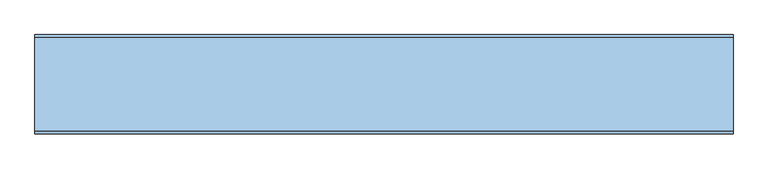
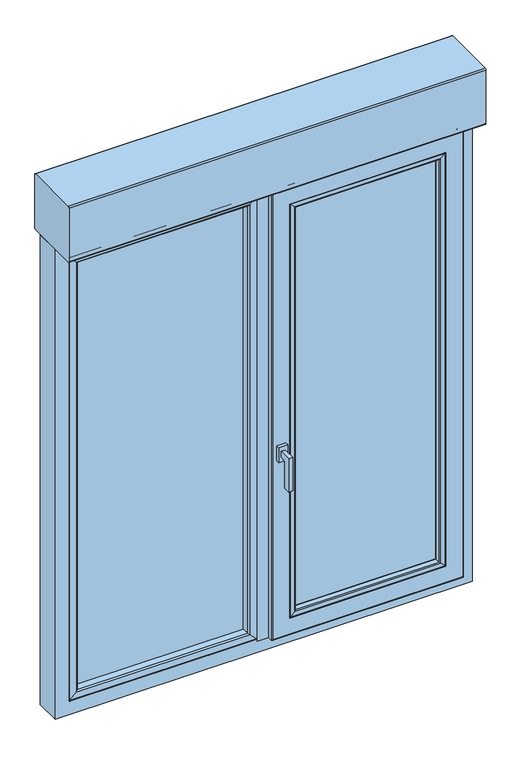
"""IFC4 building model written with IfcOpenShell, lengths in millimetres: window geometry, 2019_ES_Ventana_Replus_re80pvc301_11103_box_1-Hoja_Panel-Fijo-Lateral_con-Compacto : 2019_ES_Ventana_replus_re80pvc_301_dormitorio_1."""

from ifc_helpers import new_model, si_unit, point, frame, frame_2d, origin, place, context, project, spatial, polyline, circle_curve, ellipse_curve, trimmed, segment, composite_curve, outline, extrude, source, transform, mapped, element, save
from ifc_brep_helpers import plane_surface, cylinder_surface, advanced_brep


def window_05755cfc(model_context):
    return source(origin(), model_context, "Body", "SolidModel", [
        extrude(outline(composite_curve([segment(polyline([(55.0, 2360.0), (-120.0, 2360.0)]), True, "CONTINUOUS"), segment(trimmed(circle_curve(frame_2d((-120.0, 2365.0)), 5.0), [point((-120.0, 2360.0))], [point((-125.0, 2365.0))], False, "CARTESIAN"), True, "CONTINUOUS"), segment(polyline([(-125.0, 2365.0), (-125.0, 2540.0)]), True, "CONTINUOUS"), segment(trimmed(circle_curve(frame_2d((-120.0, 2540.0)), 5.0), [point((-125.0, 2540.0))], [point((-120.0, 2545.0))], False, "CARTESIAN"), True, "CONTINUOUS"), segment(polyline([(-120.0, 2545.0), (55.0, 2545.0)]), True, "CONTINUOUS"), segment(trimmed(circle_curve(frame_2d((55.0, 2540.0)), 5.0), [point((55.0, 2545.0))], [point((60.0, 2540.0))], False, "CARTESIAN"), True, "CONTINUOUS"), segment(polyline([(60.0, 2540.0), (60.0, 2365.0)]), True, "CONTINUOUS"), segment(trimmed(circle_curve(frame_2d((55.0, 2365.0)), 5.0), [point((60.0, 2365.0))], [point((55.0, 2360.0))], False, "CARTESIAN"), True, "CONTINUOUS")], self_intersect=False)), frame((-650.0, 0.0, 0.0), z_axis=(1.0, 0.0, 0.0), x_axis=(0.0, 1.0, 0.0)), (0.0, 0.0, 1.0), 1300.0),
        extrude(outline(polyline([(-78.4999991, 1470.0), (-78.4999991, 1450.0), (-98.4999991, 1450.0), (-98.4999991, 1360.0), (-118.4999991, 1360.0), (-118.4999991, 1470.0), (-78.4999991, 1470.0)])), frame((38.5, 0.0, 0.0), z_axis=(1.0, 0.0, 0.0), x_axis=(0.0, 1.0, 0.0)), (0.0, 0.0, 1.0), 12.0),
        extrude(outline(polyline([(58.7312385, -78.4999991), (30.2687615, -78.4999991), (30.2687615, -68.4999991), (58.7312385, -68.4999991), (58.7312385, -78.4999991)])), frame((0.0, 0.0, 1435.217127), z_axis=(0.0, 0.0, 1.0), x_axis=(1.0, 0.0, 0.0)), (0.0, 0.0, 1.0), 49.565746),
        advanced_brep(
        [(-22.1502489, -49.9816666, 2314.0497511), (-41.8192398, -49.2838062, 2294.3807602), (-41.8192398, -49.2838062, 875.6192398), (-22.1502489, -49.9816666, 855.9502489), (-46.4697163, -45.5846502, 2289.7302837), (-46.4697163, -45.5846502, 880.2697163), (-584.3807594, -49.2838062, 875.6192398), (-604.0497503, -49.9816666, 855.9502489), (-21.0, -48.871505, 2315.2), (-21.0, -48.871505, 854.8), (-51.0475336, -28.5000036, 2285.1524664), (-51.0475336, -28.5000036, 884.8475336), (-579.7302829, -45.5846502, 880.2697163), (-43.2922784, -28.5000036, 877.0922784), (-582.9077208, -28.5000036, 877.0922784), (-582.9077208, -28.5000036, 2292.9077216), (-43.2922784, -28.5000036, 2292.9077216), (-575.1524657, -28.5000036, 2285.1524664), (-575.1524657, -28.5000036, 884.8475336), (-35.4855, -36.306782, 2300.7145), (-35.4855, -36.306782, 869.2855), (-35.4855, -39.5069121, 2300.7145), (-35.4855, -39.5069121, 869.2855), (-590.7144993, -36.306782, 869.2855), (-21.0, -39.5069121, 854.8), (-605.1999993, -39.5069121, 854.8), (-605.1999993, -39.5069121, 2315.2), (-21.0, -39.5069121, 2315.2), (-590.7144993, -39.5069121, 2300.7145), (-590.7144993, -39.5069121, 869.2855), (-605.1999993, -48.871505, 854.8), (-584.3807594, -49.2838062, 2294.3807602), (-604.0497503, -49.9816666, 2314.0497511), (-579.7302829, -45.5846502, 2289.7302837), (-590.7144993, -36.306782, 2300.7145), (-605.1999993, -48.871505, 2315.2)],
        [
            (0, 1),
            (1, 2),
            (2, 3),
            (3, 0),
            (1, 4, ellipse_curve(frame((-41.6449168, -44.2918491, 2294.5550832), z_axis=(0.7071067811865475, 0.0, -0.7071067811865475), x_axis=(0.7071067811865474, 0.0, 0.7071067811865476)), 7.0639967, 4.995)),
            (4, 5),
            (5, 2, ellipse_curve(frame((-41.6449168, -44.2918491, 875.4449168), z_axis=(0.7071067811865475, 0.0, 0.7071067811865475), x_axis=(-0.7071067811865474, 0.0, 0.7071067811865476)), 7.0639967, 4.995)),
            (2, 6),
            (6, 7),
            (7, 3),
            (8, 0, ellipse_curve(frame((-22.1108601, -48.871505, 2314.0891399), z_axis=(0.7071067811865475, 0.0, -0.7071067811865475), x_axis=(0.7071067811865474, 0.0, 0.7071067811865476)), 1.5709935, 1.1108601)),
            (3, 9, ellipse_curve(frame((-22.1108601, -48.871505, 855.9108601), z_axis=(0.7071067811865475, 0.0, 0.7071067811865475), x_axis=(-0.7071067811865474, 0.0, 0.7071067811865476)), 1.5709935, 1.1108601)),
            (9, 8),
            (4, 10),
            (10, 11),
            (11, 5),
            (5, 12),
            (12, 6, ellipse_curve(frame((-584.5550824, -44.2918491, 875.4449168), z_axis=(0.7071067811865475, 0.0, -0.7071067811865475), x_axis=(0.7071067811865476, 0.0, 0.7071067811865474)), 7.0639967, 4.995)),
            (13, 14),
            (14, 15),
            (15, 16),
            (16, 13),
            (10, 17),
            (17, 18),
            (18, 11),
            (18, 12),
            (16, 19),
            (19, 20),
            (20, 13),
            (19, 21),
            (21, 22),
            (22, 20),
            (20, 23),
            (23, 14),
            (24, 25),
            (25, 26),
            (26, 27),
            (27, 24),
            (21, 28),
            (28, 29),
            (29, 22),
            (29, 23),
            (9, 24),
            (27, 8),
            (9, 30),
            (30, 25),
            (7, 30, ellipse_curve(frame((-604.0891391, -48.871505, 855.9108601), z_axis=(0.7071067811865475, 0.0, -0.7071067811865475), x_axis=(0.7071067811865476, 0.0, 0.7071067811865474)), 1.5709935, 1.1108601)),
            (6, 31),
            (31, 32),
            (32, 7),
            (12, 33),
            (33, 31, ellipse_curve(frame((-584.5550824, -44.2918491, 2294.5550832), z_axis=(-0.7071067811865475, 0.0, -0.7071067811865475), x_axis=(0.7071067811865474, 0.0, -0.7071067811865476)), 7.0639967, 4.995)),
            (17, 33),
            (23, 34),
            (34, 15),
            (28, 34),
            (30, 35),
            (35, 26),
            (32, 35, ellipse_curve(frame((-604.0891391, -48.871505, 2314.0891399), z_axis=(-0.7071067811865475, 0.0, -0.7071067811865475), x_axis=(0.7071067811865474, 0.0, -0.7071067811865476)), 1.5709935, 1.1108601)),
            (31, 1),
            (0, 32),
            (33, 4),
            (34, 19),
            (35, 8),
        ],
        [
            plane_surface(frame((-41.8192398, -49.2838062, 2294.3807602), z_axis=(-0.03545791932093323, -0.9993711702652975, 0.0), x_axis=(0.0, 0.0, -1.0))),
            cylinder_surface(frame((-41.6449168, -44.2918491, 2322.2), z_axis=(0.0, 0.0, 1.0), x_axis=(-1.0, 0.0, 0.0)), 4.995),
            plane_surface(frame((-41.8192398, -49.2838062, 875.6192398), z_axis=(0.0, -0.9993711702652976, 0.03545791932093001), x_axis=(-1.0, 0.0, 0.0))),
            cylinder_surface(frame((-22.1108601, -48.871505, 2322.2), z_axis=(0.0, 0.0, 1.0), x_axis=(-1.0, 0.0, 0.0)), 1.1108601),
            plane_surface(frame((-51.0475336, -28.5000036, 2285.1524664), z_axis=(-0.9659258262890638, -0.25881904510253767, 0.0), x_axis=(0.0, 0.0, -1.0))),
            cylinder_surface(frame((-14.0, -44.2918491, 875.4449168), z_axis=(1.0, 0.0, 0.0), x_axis=(0.0, 0.0, 1.0)), 4.995),
            plane_surface(frame((-582.9077208, -28.5000036, 2292.9077216), z_axis=(0.0, 1.0, 0.0), x_axis=(1.0, 0.0, 0.0))),
            plane_surface(frame((-51.0475336, -28.5000036, 884.8475336), z_axis=(0.0, -0.25881904510254083, 0.965925826289063), x_axis=(-1.0, 0.0, 0.0))),
            plane_surface(frame((-35.4855, -36.306782, 2300.7145), z_axis=(0.7071067811865617, 0.7071067811865334, 0.0), x_axis=(0.0, 0.0, -1.0))),
            plane_surface(frame((-35.4855, -39.5069121, 2300.7145), z_axis=(1.0, 0.0, 0.0), x_axis=(0.0, 0.0, -1.0))),
            plane_surface(frame((-35.4855, -36.306782, 869.2855), z_axis=(0.0, 0.7071067811865357, -0.7071067811865593), x_axis=(-1.0, 0.0, 0.0))),
            plane_surface(frame((-605.1999993, -39.5069121, 2315.2), z_axis=(0.0, 1.0, 0.0), x_axis=(1.0, 0.0, 0.0))),
            plane_surface(frame((-35.4855, -39.5069121, 869.2855), z_axis=(0.0, 0.0, -1.0), x_axis=(-1.0, 0.0, 0.0))),
            plane_surface(frame((-21.0, -46.2002121, 2315.2), z_axis=(1.0, 0.0, 0.0), x_axis=(0.0, 0.0, -1.0))),
            plane_surface(frame((-21.0, -46.2002121, 854.8), z_axis=(0.0, 0.0, -1.0), x_axis=(-1.0, 0.0, 0.0))),
            cylinder_surface(frame((-14.0, -48.871505, 855.9108601), z_axis=(1.0, 0.0, 0.0), x_axis=(0.0, 0.0, 1.0)), 1.1108601),
            plane_surface(frame((-584.3807594, -49.2838062, 875.6192398), z_axis=(0.03545791932092679, -0.9993711702652978, 0.0), x_axis=(0.0, 0.0, 1.0))),
            cylinder_surface(frame((-584.5550824, -44.2918491, 847.8), z_axis=(0.0, 0.0, -1.0), x_axis=(1.0, 0.0, 0.0)), 4.995),
            plane_surface(frame((-575.1524657, -28.5000036, 884.8475336), z_axis=(0.9659258262890621, -0.25881904510254394, 0.0), x_axis=(0.0, 0.0, 1.0))),
            plane_surface(frame((-590.7144993, -36.306782, 869.2855), z_axis=(-0.707106781186557, 0.707106781186538, 0.0), x_axis=(0.0, 0.0, 1.0))),
            plane_surface(frame((-590.7144993, -39.5069121, 869.2855), z_axis=(-1.0, 0.0, 0.0), x_axis=(0.0, 0.0, 1.0))),
            plane_surface(frame((-605.1999993, -46.2002121, 854.8), z_axis=(-1.0, 0.0, 0.0), x_axis=(0.0, 0.0, 1.0))),
            cylinder_surface(frame((-604.0891391, -48.871505, 847.8), z_axis=(0.0, 0.0, -1.0), x_axis=(1.0, 0.0, 0.0)), 1.1108601),
            plane_surface(frame((-584.3807594, -49.2838062, 2294.3807602), z_axis=(0.0, -0.9993711702652976, -0.03545791932093001), x_axis=(1.0, 0.0, 0.0))),
            cylinder_surface(frame((-612.1999993, -44.2918491, 2294.5550832), z_axis=(-1.0, 0.0, 0.0), x_axis=(0.0, 0.0, -1.0)), 4.995),
            plane_surface(frame((-575.1524657, -28.5000036, 2285.1524664), z_axis=(0.0, -0.25881904510254083, -0.965925826289063), x_axis=(1.0, 0.0, 0.0))),
            plane_surface(frame((-590.7144993, -36.306782, 2300.7145), z_axis=(0.0, 0.7071067811865357, 0.7071067811865593), x_axis=(1.0, 0.0, 0.0))),
            plane_surface(frame((-590.7144993, -39.5069121, 2300.7145), z_axis=(0.0, 0.0, 1.0), x_axis=(1.0, 0.0, 0.0))),
            plane_surface(frame((-605.1999993, -46.2002121, 2315.2), z_axis=(0.0, 0.0, 1.0), x_axis=(1.0, 0.0, 0.0))),
            cylinder_surface(frame((-612.1999993, -48.871505, 2314.0891399), z_axis=(-1.0, 0.0, 0.0), x_axis=(0.0, 0.0, -1.0)), 1.1108601),
        ],
        [
            (0, [[1, 2, 3, 4]]),
            (1, [[5, 6, 7, -2]]),
            (2, [[-3, 8, 9, 10]]),
            (3, [[11, -4, 12, 13]]),
            (4, [[14, 15, 16, -6]]),
            (5, [[-7, 17, 18, -8]]),
            (6, [[19, 20, 21, 22], [23, 24, 25, -15]]),
            (7, [[-16, -25, 26, -17]]),
            (8, [[27, 28, 29, -22]]),
            (9, [[30, 31, 32, -28]]),
            (10, [[-29, 33, 34, -19]]),
            (11, [[35, 36, 37, 38], [39, 40, 41, -31]]),
            (12, [[-32, -41, 42, -33]]),
            (13, [[-13, 43, -38, 44]]),
            (14, [[-43, 45, 46, -35]]),
            (15, [[-12, -10, 47, -45]]),
            (16, [[-9, 48, 49, 50]]),
            (17, [[-18, 51, 52, -48]]),
            (18, [[-26, -24, 53, -51]]),
            (19, [[-34, 54, 55, -20]]),
            (20, [[-42, -40, 56, -54]]),
            (21, [[-46, 57, 58, -36]]),
            (22, [[-47, -50, 59, -57]]),
            (23, [[-49, 60, -1, 61]]),
            (24, [[-52, 62, -5, -60]]),
            (25, [[-53, -23, -14, -62]]),
            (26, [[-55, 63, -27, -21]]),
            (27, [[-56, -39, -30, -63]]),
            (28, [[-58, 64, -44, -37]]),
            (29, [[-59, -61, -11, -64]]),
        ],
    ),
        advanced_brep(
        [(48.1911809, 11.5, 2290.2), (48.1911809, 11.5, 879.8), (48.1911809, -11.9999991, 879.8), (48.1911809, -11.9999991, 2290.2), (580.1999993, 11.5, 2290.2), (580.1999993, 11.5, 879.8), (88.2020856, 11.5, 919.8109047), (540.1890945, 11.5, 919.8109047), (540.1890945, 11.5, 2250.1890953), (88.2020856, 11.5, 2250.1890953), (580.1999993, -11.9999991, 879.8), (35.1911809, -11.9999991, 2303.2), (593.1999993, -11.9999991, 2303.2), (593.1999993, -11.9999991, 866.8), (35.1911809, -11.9999991, 866.8), (580.1999993, -11.9999991, 2290.2), (35.1911809, -50.0, 866.8), (35.1911809, -50.0, 2303.2), (593.1999993, -50.0, 866.8), (15.1911809, -50.0, 2323.2), (613.1999993, -50.0, 2323.2), (613.1999993, -50.0, 846.8), (15.1911809, -50.0, 846.8), (593.1999993, -50.0, 2303.2), (15.1911809, -65.4999991, 2323.2), (15.1911809, -65.4999991, 846.8), (613.1999993, -65.4999991, 846.8), (18.1911809, -68.4999991, 2320.2), (18.1911809, -68.4999991, 849.8), (610.1999993, -68.4999991, 849.8), (610.1999993, -68.4999991, 2320.2), (70.9541209, -68.4999991, 2267.43706), (557.4370593, -68.4999991, 2267.43706), (557.4370593, -68.4999991, 902.56294), (70.9541209, -68.4999991, 902.56294), (72.1911809, -67.2629391, 2266.2), (72.1911809, -67.2629391, 903.8), (556.1999993, -67.2629391, 903.8), (72.7423375, -67.7951848, 2265.6488434), (72.7423375, -67.7951848, 904.3511566), (555.6488427, -67.7951848, 904.3511566), (85.7676831, -67.3403297, 2252.6234978), (85.7676831, -67.3403297, 917.3765022), (542.6234971, -67.3403297, 917.3765022), (89.4917884, -64.3780426, 2248.8993925), (89.4917884, -64.3780426, 921.1006075), (538.8993918, -64.3780426, 921.1006075), (92.8970803, -51.6693201, 2245.4941006), (92.8970803, -51.6693201, 924.5058994), (535.4940999, -51.6693201, 924.5058994), (92.3834932, -51.0000003, 2246.0076877), (92.3834932, -51.0000003, 923.9923123), (536.007687, -51.0000003, 923.9923123), (81.1911809, -51.0000003, 2257.2), (547.1999993, -51.0000003, 2257.2), (547.1999993, -51.0000003, 912.8), (81.1911809, -51.0000003, 912.8), (536.007687, -51.0000003, 2246.0076877), (81.1911809, -56.4999995, 2257.2), (81.1911809, -56.4999995, 912.8), (547.1999993, -56.4999995, 912.8), (69.1911809, -56.4999995, 2269.2), (559.1999993, -56.4999995, 2269.2), (559.1999993, -56.4999995, 900.8), (69.1911809, -56.4999995, 900.8), (547.1999993, -56.4999995, 2257.2), (69.1911809, -25.6153717, 2269.2), (69.1911809, -25.6153717, 900.8), (559.1999993, -25.6153717, 900.8), (66.574961, -6.9999997, 2271.8162199), (66.574961, -6.9999997, 898.1837801), (561.8162192, -6.9999997, 898.1837801), (561.8162192, -6.9999997, 2271.8162199), (87.1911809, -6.9999997, 2251.2), (541.1999993, -6.9999997, 2251.2), (541.1999993, -6.9999997, 918.8), (87.1911809, -6.9999997, 918.8), (87.1911809, -3.0000033, 2251.2), (87.1911809, -3.0000033, 918.8), (541.1999993, -3.0000033, 918.8), (541.1999993, -3.0000033, 2251.2), (93.7172496, -3.0000033, 2244.6739313), (534.6739305, -3.0000033, 2244.6739313), (534.6739305, -3.0000033, 925.3260687), (93.7172496, -3.0000033, 925.3260687), (94.2153834, -2.3508228, 2244.1757976), (94.2153834, -2.3508228, 925.8242024), (534.1757968, -2.3508228, 925.8242024), (91.0998631, 9.2764571, 2247.2913178), (91.0998631, 9.2764571, 922.7086822), (537.2913171, 9.2764571, 922.7086822), (613.1999993, -65.4999991, 2323.2), (556.1999993, -67.2629391, 2266.2), (555.6488427, -67.7951848, 2265.6488434), (542.6234971, -67.3403297, 2252.6234978), (538.8993918, -64.3780426, 2248.8993925), (535.4940999, -51.6693201, 2245.4941006), (559.1999993, -25.6153717, 2269.2), (534.1757968, -2.3508228, 2244.1757976), (537.2913171, 9.2764571, 2247.2913178)],
        [
            (0, 1),
            (1, 2),
            (2, 3),
            (3, 0),
            (0, 4),
            (4, 5),
            (5, 1),
            (6, 7),
            (7, 8),
            (8, 9),
            (9, 6),
            (5, 10),
            (10, 2),
            (11, 12),
            (12, 13),
            (13, 14),
            (14, 11),
            (10, 15),
            (15, 3),
            (14, 16),
            (16, 17),
            (17, 11),
            (13, 18),
            (18, 16),
            (19, 20),
            (20, 21),
            (21, 22),
            (22, 19),
            (18, 23),
            (23, 17),
            (24, 19),
            (22, 25),
            (25, 24),
            (21, 26),
            (26, 25),
            (27, 24, ellipse_curve(frame((18.1911809, -65.4999991, 2320.2), z_axis=(-0.7071067811865475, 0.0, -0.7071067811865475), x_axis=(-0.7071067811865474, 0.0, 0.7071067811865476)), 4.2426407, 3.0)),
            (25, 28, ellipse_curve(frame((18.1911809, -65.4999991, 849.8), z_axis=(-0.7071067811865475, 0.0, 0.7071067811865475), x_axis=(0.7071067811865474, 0.0, 0.7071067811865476)), 4.2426407, 3.0)),
            (28, 27),
            (26, 29, ellipse_curve(frame((610.1999993, -65.4999991, 849.8), z_axis=(-0.7071067811865475, 0.0, -0.7071067811865475), x_axis=(-0.7071067811865476, 0.0, 0.7071067811865474)), 4.2426407, 3.0)),
            (29, 28),
            (29, 30),
            (30, 27),
            (31, 32),
            (32, 33),
            (33, 34),
            (34, 31),
            (35, 31, ellipse_curve(frame((70.9541209, -67.2629391, 2267.43706), z_axis=(-0.7071067811865475, 0.0, -0.7071067811865475), x_axis=(-0.7071067811865474, 0.0, 0.7071067811865476)), 1.7494671, 1.23706)),
            (34, 36, ellipse_curve(frame((70.9541209, -67.2629391, 902.56294), z_axis=(-0.7071067811865475, 0.0, 0.7071067811865475), x_axis=(0.7071067811865474, 0.0, 0.7071067811865476)), 1.7494671, 1.23706)),
            (36, 35),
            (33, 37, ellipse_curve(frame((557.4370593, -67.2629391, 902.56294), z_axis=(-0.7071067811865475, 0.0, -0.7071067811865475), x_axis=(-0.7071067811865476, 0.0, 0.7071067811865474)), 1.7494671, 1.23706)),
            (37, 36),
            (38, 35, ellipse_curve(frame((72.7237511, -67.2629391, 2265.6674299), z_axis=(-0.7071067811865475, 0.0, -0.7071067811865475), x_axis=(-0.7071067811865474, 0.0, 0.7071067811865476)), 0.7531679, 0.5325701)),
            (36, 39, ellipse_curve(frame((72.7237511, -67.2629391, 904.3325701), z_axis=(-0.7071067811865475, 0.0, 0.7071067811865475), x_axis=(0.7071067811865474, 0.0, 0.7071067811865476)), 0.7531679, 0.5325701)),
            (39, 38),
            (37, 40, ellipse_curve(frame((555.6674291, -67.2629391, 904.3325701), z_axis=(-0.7071067811865475, 0.0, -0.7071067811865475), x_axis=(-0.7071067811865476, 0.0, 0.7071067811865474)), 0.7531679, 0.5325701)),
            (40, 39),
            (41, 38),
            (39, 42),
            (42, 41),
            (40, 43),
            (43, 42),
            (44, 41, ellipse_curve(frame((85.6280851, -63.3427664, 2252.7630958), z_axis=(-0.7071067811865475, 0.0, -0.7071067811865475), x_axis=(-0.7071067811865474, 0.0, 0.7071067811865476)), 5.6568542, 4.0)),
            (42, 45, ellipse_curve(frame((85.6280851, -63.3427664, 917.2369042), z_axis=(-0.7071067811865475, 0.0, 0.7071067811865475), x_axis=(0.7071067811865474, 0.0, 0.7071067811865476)), 5.6568542, 4.0)),
            (45, 44),
            (43, 46, ellipse_curve(frame((542.7630951, -63.3427664, 917.2369042), z_axis=(-0.7071067811865475, 0.0, -0.7071067811865475), x_axis=(-0.7071067811865476, 0.0, 0.7071067811865474)), 5.6568542, 4.0)),
            (46, 45),
            (47, 44),
            (45, 48),
            (48, 47),
            (46, 49),
            (49, 48),
            (50, 47, ellipse_curve(frame((92.3834932, -51.5317048, 2246.0076877), z_axis=(-0.7071067811865475, 0.0, -0.7071067811865475), x_axis=(-0.7071067811865474, 0.0, 0.7071067811865476)), 0.7519437, 0.5317045)),
            (48, 51, ellipse_curve(frame((92.3834932, -51.5317048, 923.9923123), z_axis=(-0.7071067811865475, 0.0, 0.7071067811865475), x_axis=(0.7071067811865474, 0.0, 0.7071067811865476)), 0.7519437, 0.5317045)),
            (51, 50),
            (49, 52, ellipse_curve(frame((536.007687, -51.5317048, 923.9923123), z_axis=(-0.7071067811865475, 0.0, -0.7071067811865475), x_axis=(-0.7071067811865476, 0.0, 0.7071067811865474)), 0.7519437, 0.5317045)),
            (52, 51),
            (53, 54),
            (54, 55),
            (55, 56),
            (56, 53),
            (52, 57),
            (57, 50),
            (58, 53),
            (56, 59),
            (59, 58),
            (55, 60),
            (60, 59),
            (61, 62),
            (62, 63),
            (63, 64),
            (64, 61),
            (60, 65),
            (65, 58),
            (66, 61),
            (64, 67),
            (67, 66),
            (63, 68),
            (68, 67),
            (69, 66),
            (67, 70),
            (70, 69),
            (68, 71),
            (71, 70),
            (71, 72),
            (72, 69),
            (73, 74),
            (74, 75),
            (75, 76),
            (76, 73),
            (77, 73),
            (76, 78),
            (78, 77),
            (75, 79),
            (79, 78),
            (79, 80),
            (80, 77),
            (81, 82),
            (82, 83),
            (83, 84),
            (84, 81),
            (85, 81, ellipse_curve(frame((93.7172496, -2.4842973, 2244.6739313), z_axis=(-0.7071067811865475, 0.0, -0.7071067811865475), x_axis=(-0.7071067811865474, 0.0, 0.7071067811865476)), 0.7293184, 0.515706)),
            (84, 86, ellipse_curve(frame((93.7172496, -2.4842973, 925.3260687), z_axis=(-0.7071067811865475, 0.0, 0.7071067811865475), x_axis=(0.7071067811865474, 0.0, 0.7071067811865476)), 0.7293184, 0.515706)),
            (86, 85),
            (83, 87, ellipse_curve(frame((534.6739305, -2.4842973, 925.3260687), z_axis=(-0.7071067811865475, 0.0, -0.7071067811865475), x_axis=(-0.7071067811865476, 0.0, 0.7071067811865474)), 0.7293184, 0.515706)),
            (87, 86),
            (88, 85),
            (86, 89),
            (89, 88),
            (87, 90),
            (90, 89),
            (9, 88, ellipse_curve(frame((88.2020856, 8.5, 2250.1890953), z_axis=(-0.7071067811865475, 0.0, -0.7071067811865475), x_axis=(-0.7071067811865474, 0.0, 0.7071067811865476)), 4.2426407, 3.0)),
            (89, 6, ellipse_curve(frame((88.2020856, 8.5, 919.8109047), z_axis=(-0.7071067811865475, 0.0, 0.7071067811865475), x_axis=(0.7071067811865474, 0.0, 0.7071067811865476)), 4.2426407, 3.0)),
            (90, 7, ellipse_curve(frame((540.1890945, 8.5, 919.8109047), z_axis=(-0.7071067811865475, 0.0, -0.7071067811865475), x_axis=(-0.7071067811865476, 0.0, 0.7071067811865474)), 4.2426407, 3.0)),
            (4, 15),
            (12, 23),
            (20, 91),
            (91, 26),
            (91, 30, ellipse_curve(frame((610.1999993, -65.4999991, 2320.2), z_axis=(0.7071067811865475, 0.0, -0.7071067811865475), x_axis=(-0.7071067811865474, 0.0, -0.7071067811865476)), 4.2426407, 3.0)),
            (32, 92, ellipse_curve(frame((557.4370593, -67.2629391, 2267.43706), z_axis=(0.7071067811865475, 0.0, -0.7071067811865475), x_axis=(-0.7071067811865474, 0.0, -0.7071067811865476)), 1.7494671, 1.23706)),
            (92, 37),
            (92, 93, ellipse_curve(frame((555.6674291, -67.2629391, 2265.6674299), z_axis=(0.7071067811865475, 0.0, -0.7071067811865475), x_axis=(-0.7071067811865474, 0.0, -0.7071067811865476)), 0.7531679, 0.5325701)),
            (93, 40),
            (93, 94),
            (94, 43),
            (94, 95, ellipse_curve(frame((542.7630951, -63.3427664, 2252.7630958), z_axis=(0.7071067811865475, 0.0, -0.7071067811865475), x_axis=(-0.7071067811865474, 0.0, -0.7071067811865476)), 5.6568542, 4.0)),
            (95, 46),
            (95, 96),
            (96, 49),
            (96, 57, ellipse_curve(frame((536.007687, -51.5317048, 2246.0076877), z_axis=(0.7071067811865475, 0.0, -0.7071067811865475), x_axis=(-0.7071067811865474, 0.0, -0.7071067811865476)), 0.7519437, 0.5317045)),
            (54, 65),
            (62, 97),
            (97, 68),
            (97, 72),
            (74, 80),
            (82, 98, ellipse_curve(frame((534.6739305, -2.4842973, 2244.6739313), z_axis=(0.7071067811865475, 0.0, -0.7071067811865475), x_axis=(-0.7071067811865474, 0.0, -0.7071067811865476)), 0.7293184, 0.515706)),
            (98, 87),
            (98, 99),
            (99, 90),
            (99, 8, ellipse_curve(frame((540.1890945, 8.5, 2250.1890953), z_axis=(0.7071067811865475, 0.0, -0.7071067811865475), x_axis=(-0.7071067811865474, 0.0, -0.7071067811865476)), 4.2426407, 3.0)),
            (24, 91),
            (35, 92),
            (38, 93),
            (41, 94),
            (44, 95),
            (47, 96),
            (66, 97),
            (85, 98),
            (88, 99),
        ],
        [
            plane_surface(frame((48.1911809, -1.4999991, 2290.2), z_axis=(-1.0, 0.0, 0.0), x_axis=(0.0, 0.0, -1.0))),
            plane_surface(frame((540.1890945, 11.5, 2250.1890953), z_axis=(0.0, 1.0, 0.0), x_axis=(-1.0, 0.0, 0.0))),
            plane_surface(frame((48.1911809, -1.4999991, 879.8), z_axis=(0.0, 0.0, -1.0), x_axis=(1.0, 0.0, 0.0))),
            plane_surface(frame((585.7000002, -11.9999991, 2295.7000009), z_axis=(0.0, 1.0, 0.0), x_axis=(-1.0, 0.0, 0.0))),
            plane_surface(frame((35.1911809, -45.0999991, 2303.2), z_axis=(-1.0, 0.0, 0.0), x_axis=(0.0, 0.0, -1.0))),
            plane_surface(frame((35.1911809, -45.0999991, 866.8), z_axis=(0.0, 0.0, -1.0), x_axis=(1.0, 0.0, 0.0))),
            plane_surface(frame((609.2000019, -50.0, 2319.2000027), z_axis=(0.0, 1.0, 0.0), x_axis=(-1.0, 0.0, 0.0))),
            plane_surface(frame((15.1911809, -50.0, 2323.2), z_axis=(-1.0, 0.0, 0.0), x_axis=(0.0, 0.0, -1.0))),
            plane_surface(frame((15.1911809, -50.0, 846.8), z_axis=(0.0, 0.0, -1.0), x_axis=(1.0, 0.0, 0.0))),
            cylinder_surface(frame((18.1911809, -65.4999991, 2323.2), z_axis=(0.0, 0.0, 1.0), x_axis=(0.0, 1.0, 0.0)), 3.0),
            cylinder_surface(frame((15.1911809, -65.4999991, 849.8), z_axis=(-1.0, 0.0, 0.0), x_axis=(0.0, 1.0, 0.0)), 3.0),
            plane_surface(frame((610.1999993, -68.4999991, 2320.2), z_axis=(0.0, -1.0, 0.0), x_axis=(-1.0, 0.0, 0.0))),
            cylinder_surface(frame((70.9541209, -67.2629391, 2323.2), z_axis=(0.0, 0.0, 1.0), x_axis=(0.0, 1.0, 0.0)), 1.23706),
            cylinder_surface(frame((15.1911809, -67.2629391, 902.56294), z_axis=(-1.0, 0.0, 0.0), x_axis=(0.0, 1.0, 0.0)), 1.23706),
            cylinder_surface(frame((72.7237511, -67.2629391, 2323.2), z_axis=(0.0, 0.0, 1.0), x_axis=(0.0, 1.0, 0.0)), 0.5325701),
            cylinder_surface(frame((15.1911809, -67.2629391, 904.3325701), z_axis=(-1.0, 0.0, 0.0), x_axis=(0.0, 1.0, 0.0)), 0.5325701),
            plane_surface(frame((72.7423375, -67.7951848, 2265.6488434), z_axis=(0.03489949670249966, -0.9993908270190959, 0.0), x_axis=(0.0, 0.0, -1.0))),
            plane_surface(frame((72.7423375, -67.7951848, 904.3511566), z_axis=(0.0, -0.9993908270190958, 0.034899496702502884), x_axis=(1.0, 0.0, 0.0))),
            cylinder_surface(frame((85.6280851, -63.3427664, 2323.2), z_axis=(0.0, 0.0, 1.0), x_axis=(0.0, 1.0, 0.0)), 4.0),
            cylinder_surface(frame((15.1911809, -63.3427664, 917.2369042), z_axis=(-1.0, 0.0, 0.0), x_axis=(0.0, 1.0, 0.0)), 4.0),
            plane_surface(frame((89.4917884, -64.3780426, 2248.8993925), z_axis=(0.9659258262890643, -0.2588190451025359, 0.0), x_axis=(0.0, 0.0, -1.0))),
            plane_surface(frame((89.4917884, -64.3780426, 921.1006075), z_axis=(0.0, -0.2588190451025328, 0.9659258262890652), x_axis=(1.0, 0.0, 0.0))),
            cylinder_surface(frame((92.3834932, -51.5317048, 2323.2), z_axis=(0.0, 0.0, 1.0), x_axis=(0.0, 1.0, 0.0)), 0.5317045),
            cylinder_surface(frame((15.1911809, -51.5317048, 923.9923123), z_axis=(-1.0, 0.0, 0.0), x_axis=(0.0, 1.0, 0.0)), 0.5317045),
            plane_surface(frame((536.007687, -51.0000003, 2246.0076877), z_axis=(0.0, 1.0, 0.0), x_axis=(-1.0, 0.0, 0.0))),
            plane_surface(frame((81.1911809, -51.0000003, 2257.2), z_axis=(-1.0, 0.0, 0.0), x_axis=(0.0, 0.0, -1.0))),
            plane_surface(frame((81.1911809, -51.0000003, 912.8), z_axis=(0.0, 0.0, -1.0), x_axis=(1.0, 0.0, 0.0))),
            plane_surface(frame((547.1999993, -56.4999995, 2257.2), z_axis=(0.0, 1.0, 0.0), x_axis=(-1.0, 0.0, 0.0))),
            plane_surface(frame((69.1911809, -56.4999995, 2269.2), z_axis=(1.0, 0.0, 0.0), x_axis=(0.0, 0.0, -1.0))),
            plane_surface(frame((69.1911809, -56.4999995, 900.8), z_axis=(0.0, 0.0, 1.0), x_axis=(1.0, 0.0, 0.0))),
            plane_surface(frame((69.1911809, -25.6153717, 2269.2), z_axis=(0.9902680687415736, 0.13917310096004257, 0.0), x_axis=(0.0, 0.0, -1.0))),
            plane_surface(frame((69.1911809, -25.6153717, 900.8), z_axis=(0.0, 0.13917310096004576, 0.9902680687415731), x_axis=(1.0, 0.0, 0.0))),
            plane_surface(frame((561.8162192, -6.9999997, 2271.8162199), z_axis=(0.0, -1.0, 0.0), x_axis=(-1.0, 0.0, 0.0))),
            plane_surface(frame((87.1911809, -6.9999997, 2251.2), z_axis=(1.0, 0.0, 0.0), x_axis=(0.0, 0.0, -1.0))),
            plane_surface(frame((87.1911809, -6.9999997, 918.8), z_axis=(0.0, 0.0, 1.0), x_axis=(1.0, 0.0, 0.0))),
            plane_surface(frame((541.1999993, -3.0000033, 2251.2), z_axis=(0.0, -1.0, 0.0), x_axis=(-1.0, 0.0, 0.0))),
            cylinder_surface(frame((93.7172496, -2.4842973, 2323.2), z_axis=(0.0, 0.0, 1.0), x_axis=(0.0, 1.0, 0.0)), 0.515706),
            cylinder_surface(frame((15.1911809, -2.4842973, 925.3260687), z_axis=(-1.0, 0.0, 0.0), x_axis=(0.0, 1.0, 0.0)), 0.515706),
            plane_surface(frame((94.2153834, -2.3508228, 2244.1757976), z_axis=(0.9659258263570589, 0.2588190448487762, 0.0), x_axis=(0.0, 0.0, -1.0))),
            plane_surface(frame((94.2153834, -2.3508228, 925.8242024), z_axis=(0.0, 0.2588190448487794, 0.9659258263570581), x_axis=(1.0, 0.0, 0.0))),
            cylinder_surface(frame((88.2020856, 8.5, 2323.2), z_axis=(0.0, 0.0, 1.0), x_axis=(0.0, 1.0, 0.0)), 3.0),
            cylinder_surface(frame((15.1911809, 8.5, 919.8109047), z_axis=(-1.0, 0.0, 0.0), x_axis=(0.0, 1.0, 0.0)), 3.0),
            plane_surface(frame((580.1999993, -1.4999991, 879.8), z_axis=(1.0, 0.0, 0.0), x_axis=(0.0, 0.0, 1.0))),
            plane_surface(frame((593.1999993, -45.0999991, 866.8), z_axis=(1.0, 0.0, 0.0), x_axis=(0.0, 0.0, 1.0))),
            plane_surface(frame((613.1999993, -50.0, 846.8), z_axis=(1.0, 0.0, 0.0), x_axis=(0.0, 0.0, 1.0))),
            cylinder_surface(frame((610.1999993, -65.4999991, 846.8), z_axis=(0.0, 0.0, -1.0), x_axis=(0.0, 1.0, 0.0)), 3.0),
            cylinder_surface(frame((557.4370593, -67.2629391, 846.8), z_axis=(0.0, 0.0, -1.0), x_axis=(0.0, 1.0, 0.0)), 1.23706),
            cylinder_surface(frame((555.6674291, -67.2629391, 846.8), z_axis=(0.0, 0.0, -1.0), x_axis=(0.0, 1.0, 0.0)), 0.5325701),
            plane_surface(frame((555.6488427, -67.7951848, 904.3511566), z_axis=(-0.03489949670250611, -0.9993908270190957, 0.0), x_axis=(0.0, 0.0, 1.0))),
            cylinder_surface(frame((542.7630951, -63.3427664, 846.8), z_axis=(0.0, 0.0, -1.0), x_axis=(0.0, 1.0, 0.0)), 4.0),
            plane_surface(frame((538.8993918, -64.3780426, 921.1006075), z_axis=(-0.965925826289066, -0.2588190451025297, 0.0), x_axis=(0.0, 0.0, 1.0))),
            cylinder_surface(frame((536.007687, -51.5317048, 846.8), z_axis=(0.0, 0.0, -1.0), x_axis=(0.0, 1.0, 0.0)), 0.5317045),
            plane_surface(frame((547.1999993, -51.0000003, 912.8), z_axis=(1.0, 0.0, 0.0), x_axis=(0.0, 0.0, 1.0))),
            plane_surface(frame((559.1999993, -56.4999995, 900.8), z_axis=(-1.0, 0.0, 0.0), x_axis=(0.0, 0.0, 1.0))),
            plane_surface(frame((559.1999993, -25.6153717, 900.8), z_axis=(-0.9902680687415727, 0.13917310096004895, 0.0), x_axis=(0.0, 0.0, 1.0))),
            plane_surface(frame((541.1999993, -6.9999997, 918.8), z_axis=(-1.0, 0.0, 0.0), x_axis=(0.0, 0.0, 1.0))),
            cylinder_surface(frame((534.6739305, -2.4842973, 846.8), z_axis=(0.0, 0.0, -1.0), x_axis=(0.0, 1.0, 0.0)), 0.515706),
            plane_surface(frame((534.1757968, -2.3508228, 925.8242024), z_axis=(-0.9659258263570573, 0.2588190448487825, 0.0), x_axis=(0.0, 0.0, 1.0))),
            cylinder_surface(frame((540.1890945, 8.5, 846.8), z_axis=(0.0, 0.0, -1.0), x_axis=(0.0, 1.0, 0.0)), 3.0),
            plane_surface(frame((580.1999993, -1.4999991, 2290.2), z_axis=(0.0, 0.0, 1.0), x_axis=(-1.0, 0.0, 0.0))),
            plane_surface(frame((593.1999993, -45.0999991, 2303.2), z_axis=(0.0, 0.0, 1.0), x_axis=(-1.0, 0.0, 0.0))),
            plane_surface(frame((613.1999993, -50.0, 2323.2), z_axis=(0.0, 0.0, 1.0), x_axis=(-1.0, 0.0, 0.0))),
            cylinder_surface(frame((613.1999993, -65.4999991, 2320.2), z_axis=(1.0, 0.0, 0.0), x_axis=(0.0, 1.0, 0.0)), 3.0),
            cylinder_surface(frame((613.1999993, -67.2629391, 2267.43706), z_axis=(1.0, 0.0, 0.0), x_axis=(0.0, 1.0, 0.0)), 1.23706),
            cylinder_surface(frame((613.1999993, -67.2629391, 2265.6674299), z_axis=(1.0, 0.0, 0.0), x_axis=(0.0, 1.0, 0.0)), 0.5325701),
            plane_surface(frame((555.6488427, -67.7951848, 2265.6488434), z_axis=(0.0, -0.9993908270190958, -0.034899496702502884), x_axis=(-1.0, 0.0, 0.0))),
            cylinder_surface(frame((613.1999993, -63.3427664, 2252.7630958), z_axis=(1.0, 0.0, 0.0), x_axis=(0.0, 1.0, 0.0)), 4.0),
            plane_surface(frame((538.8993918, -64.3780426, 2248.8993925), z_axis=(0.0, -0.2588190451025328, -0.9659258262890651), x_axis=(-1.0, 0.0, 0.0))),
            cylinder_surface(frame((613.1999993, -51.5317048, 2246.0076877), z_axis=(1.0, 0.0, 0.0), x_axis=(0.0, 1.0, 0.0)), 0.5317045),
            plane_surface(frame((547.1999993, -51.0000003, 2257.2), z_axis=(0.0, 0.0, 1.0), x_axis=(-1.0, 0.0, 0.0))),
            plane_surface(frame((559.1999993, -56.4999995, 2269.2), z_axis=(0.0, 0.0, -1.0), x_axis=(-1.0, 0.0, 0.0))),
            plane_surface(frame((559.1999993, -25.6153717, 2269.2), z_axis=(0.0, 0.13917310096004576, -0.9902680687415731), x_axis=(-1.0, 0.0, 0.0))),
            plane_surface(frame((541.1999993, -6.9999997, 2251.2), z_axis=(0.0, 0.0, -1.0), x_axis=(-1.0, 0.0, 0.0))),
            cylinder_surface(frame((613.1999993, -2.4842973, 2244.6739313), z_axis=(1.0, 0.0, 0.0), x_axis=(0.0, 1.0, 0.0)), 0.515706),
            plane_surface(frame((534.1757968, -2.3508228, 2244.1757976), z_axis=(0.0, 0.2588190448487794, -0.9659258263570581), x_axis=(-1.0, 0.0, 0.0))),
            cylinder_surface(frame((613.1999993, 8.5, 2250.1890953), z_axis=(1.0, 0.0, 0.0), x_axis=(0.0, 1.0, 0.0)), 3.0),
        ],
        [
            (0, [[1, 2, 3, 4]]),
            (1, [[5, 6, 7, -1], [8, 9, 10, 11]]),
            (2, [[-2, -7, 12, 13]]),
            (3, [[14, 15, 16, 17], [-13, 18, 19, -3]]),
            (4, [[-17, 20, 21, 22]]),
            (5, [[-20, -16, 23, 24]]),
            (6, [[25, 26, 27, 28], [-24, 29, 30, -21]]),
            (7, [[31, -28, 32, 33]]),
            (8, [[-32, -27, 34, 35]]),
            (9, [[36, -33, 37, 38]]),
            (10, [[-37, -35, 39, 40]]),
            (11, [[-40, 41, 42, -38], [43, 44, 45, 46]]),
            (12, [[47, -46, 48, 49]]),
            (13, [[-48, -45, 50, 51]]),
            (14, [[52, -49, 53, 54]]),
            (15, [[-53, -51, 55, 56]]),
            (16, [[57, -54, 58, 59]]),
            (17, [[-58, -56, 60, 61]]),
            (18, [[62, -59, 63, 64]]),
            (19, [[-63, -61, 65, 66]]),
            (20, [[67, -64, 68, 69]]),
            (21, [[-68, -66, 70, 71]]),
            (22, [[72, -69, 73, 74]]),
            (23, [[-73, -71, 75, 76]]),
            (24, [[77, 78, 79, 80], [-76, 81, 82, -74]]),
            (25, [[83, -80, 84, 85]]),
            (26, [[-84, -79, 86, 87]]),
            (27, [[88, 89, 90, 91], [-87, 92, 93, -85]]),
            (28, [[94, -91, 95, 96]]),
            (29, [[-95, -90, 97, 98]]),
            (30, [[99, -96, 100, 101]]),
            (31, [[-100, -98, 102, 103]]),
            (32, [[-103, 104, 105, -101], [106, 107, 108, 109]]),
            (33, [[110, -109, 111, 112]]),
            (34, [[-111, -108, 113, 114]]),
            (35, [[-114, 115, 116, -112], [117, 118, 119, 120]]),
            (36, [[121, -120, 122, 123]]),
            (37, [[-122, -119, 124, 125]]),
            (38, [[126, -123, 127, 128]]),
            (39, [[-127, -125, 129, 130]]),
            (40, [[131, -128, 132, -11]]),
            (41, [[-132, -130, 133, -8]]),
            (42, [[-12, -6, 134, -18]]),
            (43, [[-23, -15, 135, -29]]),
            (44, [[-34, -26, 136, 137]]),
            (45, [[-39, -137, 138, -41]]),
            (46, [[-50, -44, 139, 140]]),
            (47, [[-55, -140, 141, 142]]),
            (48, [[-60, -142, 143, 144]]),
            (49, [[-65, -144, 145, 146]]),
            (50, [[-70, -146, 147, 148]]),
            (51, [[-75, -148, 149, -81]]),
            (52, [[-86, -78, 150, -92]]),
            (53, [[-97, -89, 151, 152]]),
            (54, [[-102, -152, 153, -104]]),
            (55, [[-113, -107, 154, -115]]),
            (56, [[-124, -118, 155, 156]]),
            (57, [[-129, -156, 157, 158]]),
            (58, [[-133, -158, 159, -9]]),
            (59, [[-134, -5, -4, -19]]),
            (60, [[-135, -14, -22, -30]]),
            (61, [[-136, -25, -31, 160]]),
            (62, [[-138, -160, -36, -42]]),
            (63, [[-139, -43, -47, 161]]),
            (64, [[-141, -161, -52, 162]]),
            (65, [[-143, -162, -57, 163]]),
            (66, [[-145, -163, -62, 164]]),
            (67, [[-147, -164, -67, 165]]),
            (68, [[-149, -165, -72, -82]]),
            (69, [[-150, -77, -83, -93]]),
            (70, [[-151, -88, -94, 166]]),
            (71, [[-153, -166, -99, -105]]),
            (72, [[-154, -106, -110, -116]]),
            (73, [[-155, -117, -121, 167]]),
            (74, [[-157, -167, -126, 168]]),
            (75, [[-159, -168, -131, -10]]),
        ],
    ),
        extrude(outline(composite_curve([segment(polyline([(23.3911809, -37.9746327), (23.3911809, -49.0)]), True, "CONTINUOUS"), segment(trimmed(circle_curve(frame_2d((22.3911809, -49.0)), 1.0), [point((23.3911809, -49.0))], [point((22.3911809, -50.0))], False, "CARTESIAN"), True, "CONTINUOUS"), segment(polyline([(22.3911809, -50.0), (-19.7446784, -50.0)]), True, "CONTINUOUS"), segment(trimmed(circle_curve(frame_2d((-19.7446784, -49.0)), 1.0), [point((-19.7446784, -50.0))], [point((-20.7446784, -49.0))], False, "CARTESIAN"), True, "CONTINUOUS"), segment(polyline([(-20.7446784, -49.0), (-20.7446784, -37.9746327), (-18.5911809, -37.9746327), (-18.5911809, -8.0), (-40.6020331, -8.0), (-40.6020331, -6.2175904), (-27.9799071, 1.0697975), (-26.7556588, 15.0630198), (-41.0115567, 17.0665556), (-41.7938856, 11.4999962), (-52.5579009, 11.4999962)]), True, "CONTINUOUS"), segment(trimmed(circle_curve(frame_2d((-52.5579009, 12.4999962)), 1.0), [point((-52.5579009, 11.4999962))], [point((-53.5238267, 12.7588152))], False, "CARTESIAN"), True, "CONTINUOUS"), segment(polyline([(-53.5238267, 12.7588152), (-49.4998617, 27.7764571)]), True, "CONTINUOUS"), segment(trimmed(circle_curve(frame_2d((-46.6020842, 27.0)), 3.0), [point((-49.4998617, 27.7764571))], [point((-46.6020842, 30.0))], False, "CARTESIAN"), True, "CONTINUOUS"), segment(polyline([(-46.6020842, 30.0), (48.4020842, 30.0)]), True, "CONTINUOUS"), segment(trimmed(circle_curve(frame_2d((48.4020842, 27.0)), 3.0), [point((48.4020842, 30.0))], [point((51.2998617, 27.7764571))], False, "CARTESIAN"), True, "CONTINUOUS"), segment(polyline([(51.2998617, 27.7764571), (55.3238267, 12.7588152)]), True, "CONTINUOUS"), segment(trimmed(circle_curve(frame_2d((54.3579009, 12.4999962)), 1.0), [point((55.3238267, 12.7588152))], [point((54.3579009, 11.4999962))], False, "CARTESIAN"), True, "CONTINUOUS"), segment(polyline([(54.3579009, 11.4999962), (43.5938856, 11.4999962), (42.8115567, 17.0665556), (28.5556588, 15.0630198), (29.7799071, 1.0697975), (42.4020331, -6.2175904), (42.4020331, -8.0), (20.3911809, -8.0), (20.3911809, -37.9746327), (23.3911809, -37.9746327)]), True, "CONTINUOUS")], self_intersect=False)), frame((0.0, 0.0, 846.8), z_axis=(0.0, 0.0, 1.0), x_axis=(1.0, 0.0, 0.0)), (0.0, 0.0, 1.0), 1476.4),
        advanced_brep(
        [(606.1999993, -50.0, 2316.1999993), (605.1999993, -49.0, 2315.1999993), (605.1999993, -49.0, 854.8000007), (606.1999993, -50.0, 853.8000007), (605.1999993, -8.0, 2315.1999993), (605.1999993, -8.0, 854.8000007), (-605.1999993, -49.0, 854.8000007), (-606.1999993, -50.0, 853.8000007), (650.0, -50.0, 2360.0), (-650.0, -50.0, 2360.0), (-650.0, -50.0, 810.0), (650.0, -50.0, 810.0), (-606.1999993, -50.0, 2316.1999993), (574.2332803, 11.5, 2284.2332803), (573.2673545, 12.758819, 2283.2673545), (573.2673545, 12.758819, 886.7326455), (574.2332803, 11.5, 885.7667197), (577.2913185, 27.7764571, 2287.2913185), (577.2913185, 27.7764571, 882.7086815), (-573.2673545, 12.758819, 886.7326455), (-574.2332803, 11.5, 885.7667197), (586.1891471, 11.5, 2296.1891471), (-586.1891471, 11.5, 2296.1891471), (-586.1891471, 11.5, 873.8108529), (586.1891471, 11.5, 873.8108529), (-574.2332803, 11.5, 2284.2332803), (580.189096, 30.0, 2290.189096), (580.189096, 30.0, 879.810904), (650.0, 30.0, 810.0), (-650.0, 30.0, 810.0), (-650.0, 30.0, 2360.0), (650.0, 30.0, 2360.0), (-580.189096, 30.0, 2290.189096), (-580.189096, 30.0, 879.810904), (-577.2913185, 27.7764571, 882.7086815), (586.1891471, -8.0, 2296.1891471), (586.1891471, -8.0, 873.8108529), (-586.1891471, -8.0, 873.8108529), (-605.1999993, -8.0, 2315.1999993), (-605.1999993, -8.0, 854.8000007), (-586.1891471, -8.0, 2296.1891471), (-605.1999993, -49.0, 2315.1999993), (-573.2673545, 12.758819, 2283.2673545), (-577.2913185, 27.7764571, 2287.2913185)],
        [
            (0, 1, ellipse_curve(frame((606.1999993, -49.0, 2316.1999993), z_axis=(0.7071067811865475, 0.0, -0.7071067811865475), x_axis=(0.7071067811865474, 0.0, 0.7071067811865476)), 1.4142136, 1.0)),
            (1, 2),
            (2, 3, ellipse_curve(frame((606.1999993, -49.0, 853.8000007), z_axis=(0.7071067811865475, 0.0, 0.7071067811865475), x_axis=(-0.7071067811865474, 0.0, 0.7071067811865476)), 1.4142136, 1.0)),
            (3, 0),
            (1, 4),
            (4, 5),
            (5, 2),
            (2, 6),
            (6, 7, ellipse_curve(frame((-606.1999993, -49.0, 853.8000007), z_axis=(0.7071067811865475, 0.0, -0.7071067811865475), x_axis=(0.7071067811865476, 0.0, 0.7071067811865474)), 1.4142136, 1.0)),
            (7, 3),
            (8, 9),
            (9, 10),
            (10, 11),
            (11, 8),
            (7, 12),
            (12, 0),
            (13, 14, ellipse_curve(frame((574.2332803, 12.5, 2284.2332803), z_axis=(0.7071067811865475, 0.0, -0.7071067811865475), x_axis=(0.7071067811865474, 0.0, 0.7071067811865476)), 1.4142136, 1.0)),
            (14, 15),
            (15, 16, ellipse_curve(frame((574.2332803, 12.5, 885.7667197), z_axis=(0.7071067811865475, 0.0, 0.7071067811865475), x_axis=(-0.7071067811865474, 0.0, 0.7071067811865476)), 1.4142136, 1.0)),
            (16, 13),
            (14, 17),
            (17, 18),
            (18, 15),
            (15, 19),
            (19, 20, ellipse_curve(frame((-574.2332803, 12.5, 885.7667197), z_axis=(0.7071067811865475, 0.0, -0.7071067811865475), x_axis=(0.7071067811865476, 0.0, 0.7071067811865474)), 1.4142136, 1.0)),
            (20, 16),
            (21, 22),
            (22, 23),
            (23, 24),
            (24, 21),
            (20, 25),
            (25, 13),
            (17, 26, ellipse_curve(frame((580.189096, 27.0, 2290.189096), z_axis=(0.7071067811865475, 0.0, -0.7071067811865475), x_axis=(0.7071067811865474, 0.0, 0.7071067811865476)), 4.2426407, 3.0)),
            (26, 27),
            (27, 18, ellipse_curve(frame((580.189096, 27.0, 879.810904), z_axis=(0.7071067811865475, 0.0, 0.7071067811865475), x_axis=(-0.7071067811865474, 0.0, 0.7071067811865476)), 4.2426407, 3.0)),
            (28, 29),
            (29, 30),
            (30, 31),
            (31, 28),
            (26, 32),
            (32, 33),
            (33, 27),
            (33, 34, ellipse_curve(frame((-580.189096, 27.0, 879.810904), z_axis=(0.7071067811865475, 0.0, -0.7071067811865475), x_axis=(0.7071067811865476, 0.0, 0.7071067811865474)), 4.2426407, 3.0)),
            (34, 18),
            (34, 19),
            (35, 21),
            (24, 36),
            (36, 35),
            (23, 37),
            (37, 36),
            (4, 38),
            (38, 39),
            (39, 5),
            (37, 40),
            (40, 35),
            (31, 8),
            (11, 28),
            (10, 29),
            (39, 6),
            (6, 41),
            (41, 12, ellipse_curve(frame((-606.1999993, -49.0, 2316.1999993), z_axis=(-0.7071067811865475, 0.0, -0.7071067811865475), x_axis=(0.7071067811865474, 0.0, -0.7071067811865476)), 1.4142136, 1.0)),
            (19, 42),
            (42, 25, ellipse_curve(frame((-574.2332803, 12.5, 2284.2332803), z_axis=(-0.7071067811865475, 0.0, -0.7071067811865475), x_axis=(0.7071067811865474, 0.0, -0.7071067811865476)), 1.4142136, 1.0)),
            (32, 43, ellipse_curve(frame((-580.189096, 27.0, 2290.189096), z_axis=(-0.7071067811865475, 0.0, -0.7071067811865475), x_axis=(0.7071067811865474, 0.0, -0.7071067811865476)), 4.2426407, 3.0)),
            (43, 34),
            (43, 42),
            (22, 40),
            (9, 30),
            (38, 41),
            (41, 1),
            (42, 14),
            (17, 43),
        ],
        [
            cylinder_surface(frame((606.1999993, -49.0, 2360.0), z_axis=(0.0, 0.0, 1.0), x_axis=(-1.0, 0.0, 0.0)), 1.0),
            plane_surface(frame((605.1999993, -8.0, 2315.1999993), z_axis=(-1.0, 0.0, 0.0), x_axis=(0.0, 0.0, -1.0))),
            cylinder_surface(frame((650.0, -49.0, 853.8000007), z_axis=(1.0, 0.0, 0.0), x_axis=(0.0, 0.0, 1.0)), 1.0),
            plane_surface(frame((-606.1999993, -50.0, 2316.1999993), z_axis=(0.0, -1.0, 0.0), x_axis=(1.0, 0.0, 0.0))),
            cylinder_surface(frame((574.2332803, 12.5, 2360.0), z_axis=(0.0, 0.0, 1.0), x_axis=(-1.0, 0.0, 0.0)), 1.0),
            plane_surface(frame((577.2913185, 27.7764571, 2287.2913185), z_axis=(-0.9659258262890683, 0.25881904510252085, 0.0), x_axis=(0.0, 0.0, -1.0))),
            cylinder_surface(frame((650.0, 12.5, 885.7667197), z_axis=(1.0, 0.0, 0.0), x_axis=(0.0, 0.0, 1.0)), 1.0),
            plane_surface(frame((-574.2332803, 11.5, 2284.2332803), z_axis=(0.0, -1.0, 0.0), x_axis=(1.0, 0.0, 0.0))),
            cylinder_surface(frame((580.189096, 27.0, 2360.0), z_axis=(0.0, 0.0, 1.0), x_axis=(-1.0, 0.0, 0.0)), 3.0),
            plane_surface(frame((-650.0, 30.0, 2360.0), z_axis=(0.0, 1.0, 0.0), x_axis=(1.0, 0.0, 0.0))),
            cylinder_surface(frame((650.0, 27.0, 879.810904), z_axis=(1.0, 0.0, 0.0), x_axis=(0.0, 0.0, 1.0)), 3.0),
            plane_surface(frame((577.2913185, 27.7764571, 882.7086815), z_axis=(0.0, 0.25881904510251774, 0.9659258262890692), x_axis=(-1.0, 0.0, 0.0))),
            plane_surface(frame((586.1891471, 11.5, 2296.1891471), z_axis=(-1.0, 0.0, 0.0), x_axis=(0.0, 0.0, -1.0))),
            plane_surface(frame((586.1891471, 11.5, 873.8108529), z_axis=(0.0, 0.0, 1.0), x_axis=(-1.0, 0.0, 0.0))),
            plane_surface(frame((-586.1891471, -8.0, 2296.1891471), z_axis=(0.0, -1.0, 0.0), x_axis=(1.0, 0.0, 0.0))),
            plane_surface(frame((650.0, -50.0, 2360.0), z_axis=(1.0, 0.0, 0.0), x_axis=(0.0, 0.0, -1.0))),
            plane_surface(frame((650.0, -50.0, 810.0), z_axis=(0.0, 0.0, -1.0), x_axis=(-1.0, 0.0, 0.0))),
            plane_surface(frame((605.1999993, -8.0, 854.8000007), z_axis=(0.0, 0.0, 1.0), x_axis=(-1.0, 0.0, 0.0))),
            cylinder_surface(frame((-606.1999993, -49.0, 810.0), z_axis=(0.0, 0.0, -1.0), x_axis=(1.0, 0.0, 0.0)), 1.0),
            cylinder_surface(frame((-574.2332803, 12.5, 810.0), z_axis=(0.0, 0.0, -1.0), x_axis=(1.0, 0.0, 0.0)), 1.0),
            cylinder_surface(frame((-580.189096, 27.0, 810.0), z_axis=(0.0, 0.0, -1.0), x_axis=(1.0, 0.0, 0.0)), 3.0),
            plane_surface(frame((-577.2913185, 27.7764571, 882.7086815), z_axis=(0.96592582628907, 0.25881904510251463, 0.0), x_axis=(0.0, 0.0, 1.0))),
            plane_surface(frame((-586.1891471, 11.5, 873.8108529), z_axis=(1.0, 0.0, 0.0), x_axis=(0.0, 0.0, 1.0))),
            plane_surface(frame((-650.0, -50.0, 810.0), z_axis=(-1.0, 0.0, 0.0), x_axis=(0.0, 0.0, 1.0))),
            plane_surface(frame((-605.1999993, -8.0, 854.8000007), z_axis=(1.0, 0.0, 0.0), x_axis=(0.0, 0.0, 1.0))),
            cylinder_surface(frame((-650.0, -49.0, 2316.1999993), z_axis=(-1.0, 0.0, 0.0), x_axis=(0.0, 0.0, -1.0)), 1.0),
            cylinder_surface(frame((-650.0, 12.5, 2284.2332803), z_axis=(-1.0, 0.0, 0.0), x_axis=(0.0, 0.0, -1.0)), 1.0),
            cylinder_surface(frame((-650.0, 27.0, 2290.189096), z_axis=(-1.0, 0.0, 0.0), x_axis=(0.0, 0.0, -1.0)), 3.0),
            plane_surface(frame((-577.2913185, 27.7764571, 2287.2913185), z_axis=(0.0, 0.25881904510251774, -0.9659258262890692), x_axis=(1.0, 0.0, 0.0))),
            plane_surface(frame((-586.1891471, 11.5, 2296.1891471), z_axis=(0.0, 0.0, -1.0), x_axis=(1.0, 0.0, 0.0))),
            plane_surface(frame((-650.0, -50.0, 2360.0), z_axis=(0.0, 0.0, 1.0), x_axis=(1.0, 0.0, 0.0))),
            plane_surface(frame((-605.1999993, -8.0, 2315.1999993), z_axis=(0.0, 0.0, -1.0), x_axis=(1.0, 0.0, 0.0))),
        ],
        [
            (0, [[1, 2, 3, 4]]),
            (1, [[5, 6, 7, -2]]),
            (2, [[-3, 8, 9, 10]]),
            (3, [[11, 12, 13, 14], [-10, 15, 16, -4]]),
            (4, [[17, 18, 19, 20]]),
            (5, [[21, 22, 23, -18]]),
            (6, [[-19, 24, 25, 26]]),
            (7, [[27, 28, 29, 30], [-26, 31, 32, -20]]),
            (8, [[33, 34, 35, -22]]),
            (9, [[36, 37, 38, 39], [40, 41, 42, -34]]),
            (10, [[-35, -42, 43, 44]]),
            (11, [[-23, -44, 45, -24]]),
            (12, [[46, -30, 47, 48]]),
            (13, [[-47, -29, 49, 50]]),
            (14, [[51, 52, 53, -6], [-50, 54, 55, -48]]),
            (15, [[56, -14, 57, -39]]),
            (16, [[-57, -13, 58, -36]]),
            (17, [[-7, -53, 59, -8]]),
            (18, [[-9, 60, 61, -15]]),
            (19, [[-25, 62, 63, -31]]),
            (20, [[-43, -41, 64, 65]]),
            (21, [[-45, -65, 66, -62]]),
            (22, [[-49, -28, 67, -54]]),
            (23, [[-58, -12, 68, -37]]),
            (24, [[-59, -52, 69, -60]]),
            (25, [[-61, 70, -1, -16]]),
            (26, [[-63, 71, -17, -32]]),
            (27, [[-64, -40, -33, 72]]),
            (28, [[-66, -72, -21, -71]]),
            (29, [[-67, -27, -46, -55]]),
            (30, [[-68, -11, -56, -38]]),
            (31, [[-69, -51, -5, -70]]),
        ],
    ),
        extrude(outline(polyline([(-37.0063666, 11.4999962), (-37.0063666, 7.4999962), (-584.1891471, 7.4999962), (-584.1891471, 11.4999962), (-37.0063666, 11.4999962)])), frame((0.0, 0.0, 875.6108529), z_axis=(0.0, 0.0, 1.0), x_axis=(1.0, 0.0, 0.0)), (0.0, 0.0, 1.0), 1418.7782941),
        extrude(outline(polyline([(-37.0063666, -6.5), (-37.0063666, -10.5), (-584.1891471, -10.5), (-584.1891471, -6.5), (-37.0063666, -6.5)])), frame((0.0, 0.0, 875.6108529), z_axis=(0.0, 0.0, 1.0), x_axis=(1.0, 0.0, 0.0)), (0.0, 0.0, 1.0), 1418.7782941),
        extrude(outline(polyline([(-37.0063666, -24.4999997), (-37.0063666, -28.4999997), (-584.1891471, -28.4999997), (-584.1891471, -24.4999997), (-37.0063666, -24.4999997)])), frame((0.0, 0.0, 875.6108529), z_axis=(0.0, 0.0, 1.0), x_axis=(1.0, 0.0, 0.0)), (0.0, 0.0, 1.0), 1418.7782941),
        extrude(outline(polyline([(2257.0, 547.1999993), (2257.0, 81.0), (912.8, 81.0), (912.8, 547.1999993), (2257.0, 547.1999993)]), holes=[polyline([(920.8, 539.1999993), (920.8, 89.0), (2249.0, 89.0), (2249.0, 539.1999993), (920.8, 539.1999993)])]), frame((0.0, -27.0000002, 0.0), z_axis=(0.0, 1.0, 0.0), x_axis=(0.0, 0.0, 1.0)), (0.0, 0.0, 1.0), 16.0000002),
        extrude(outline(polyline([(2257.0, 547.1999993), (2257.0, 81.0), (912.8, 81.0), (912.8, 547.1999993), (2257.0, 547.1999993)]), holes=[polyline([(920.8, 539.1999993), (920.8, 89.0), (2249.0, 89.0), (2249.0, 539.1999993), (920.8, 539.1999993)])]), frame((0.0, -47.0000002, 0.0), z_axis=(0.0, 1.0, 0.0), x_axis=(0.0, 0.0, 1.0)), (0.0, 0.0, 1.0), 16.0000002),
        extrude(outline(polyline([(2288.3891471, -43.0063666), (2288.3891471, -578.1891471), (881.8608529, -578.1891471), (881.8608529, -43.0063666), (2288.3891471, -43.0063666)]), holes=[polyline([(889.8608529, -51.0063666), (889.8608529, -570.1891471), (2280.3891471, -570.1891471), (2280.3891471, -51.0063666), (889.8608529, -51.0063666)])]), frame((0.0, -24.5, 0.0), z_axis=(0.0, 1.0, 0.0), x_axis=(0.0, 0.0, 1.0)), (0.0, 0.0, 1.0), 14.0),
        extrude(outline(polyline([(2288.3891471, -43.0063666), (2288.3891471, -578.1891471), (881.8608529, -578.1891471), (881.8608529, -43.0063666), (2288.3891471, -43.0063666)]), holes=[polyline([(889.8608529, -51.0063666), (889.8608529, -570.1891471), (2280.3891471, -570.1891471), (2280.3891471, -51.0063666), (889.8608529, -51.0063666)])]), frame((0.0, -6.5, 0.0), z_axis=(0.0, 1.0, 0.0), x_axis=(0.0, 0.0, 1.0)), (0.0, 0.0, 1.0), 14.0),
        extrude(outline(polyline([(553.1999993, -6.9999997), (553.1999993, -10.9999997), (75.0, -10.9999997), (75.0, -6.9999997), (553.1999993, -6.9999997)])), frame((0.0, 0.0, 906.8), z_axis=(0.0, 0.0, 1.0), x_axis=(1.0, 0.0, 0.0)), (0.0, 0.0, 1.0), 1356.2),
        extrude(outline(polyline([(553.1999993, -26.9999997), (553.1999993, -30.9999997), (75.0, -30.9999997), (75.0, -26.9999997), (553.1999993, -26.9999997)])), frame((0.0, 0.0, 906.8), z_axis=(0.0, 0.0, 1.0), x_axis=(1.0, 0.0, 0.0)), (0.0, 0.0, 1.0), 1356.2),
        extrude(outline(polyline([(553.1999993, -46.9999997), (553.1999993, -50.9999997), (75.0, -50.9999997), (75.0, -46.9999997), (553.1999993, -46.9999997)])), frame((0.0, 0.0, 906.8), z_axis=(0.0, 0.0, 1.0), x_axis=(1.0, 0.0, 0.0)), (0.0, 0.0, 1.0), 1356.2),
    ])


if __name__ == "__main__":
    model = new_model("IFC4")
    model_context = context("Model", 3, world=origin())
    ifc_project = project(units=[si_unit("LENGTHUNIT", "METRE", prefix="MILLI")], contexts=[model_context])
    site = spatial("IfcSite", under=ifc_project)
    building = spatial("IfcBuilding", under=site)
    placement = place(None, origin())
    window_shape = window_05755cfc(model_context)
    element("IfcWindow", 1, ObjectType="2019_ES_Ventana_Replus_re80pvc301_11103_box_1-Hoja_Panel-Fijo-Lateral_con-Compacto : 2019_ES_Ventana_replus_re80pvc_301_dormitorio_1", at=placement, inside=building, context=model_context, shape_type="MappedRepresentation", body=[
        mapped(window_shape, transform((0.0, 0.0, 0.0), x_axis=(1.0, 0.0, 0.0), y_axis=(0.0, 1.0, 0.0), z_axis=(0.0, 0.0, 1.0))),
    ])
    save(model, "model.ifc")

# Revit data of these elements
# Type "2019_ES_Ventana_Replus_re80pvc301_11103_box_1-Hoja_Panel-Fijo-Lateral_con-Compacto : 2019_ES_Ventana_replus_re80pvc_301_dormitorio_1"
#   Type Mark = "48"
#   URL = "https://replus.es/"
#   Product data url = "https://bimetica.com/es/objetos-bim-replus-ventana-practicable-oscilobatiente-una-hoja-fijo-lateral-con-compacto-9544"
#   Product Guid = ""
#   Model = "11103"
#   Material secondary = "Glass"
#   Material main = "PVC"
#   Manufacturer = "Replus"
#   Keynote = "08500"
#   Description = "Perfiles de PVC con triple junta (por junta rígida en el marco). Protegiendo de este modo todos los puntos de cierre y proporcionando una junta perimetral completa, con un grosor en el perfil de 3 mm. Vidrio de alta calidad con diferentes posibilidades"
#   Assembly Code = "B2020100"
#   Analytic Construction = "<None>"
#   Ι_Wll Thcknss [instance default] = 20.0 cm
#   Ι_Wdth Cntrl = 130.0 cm
#   Ι_Nst Cntrl [instance default] = 0.0 cm
#   Ι_Hndl Hght Cntrl = 65.0 cm
#   Ι_Hght Cntrl = 155.0 cm
#   Rough Width = 132.0 cm
#   Rough Height = 157.0 cm
#   Retranqueo [instance default] = 0.0 cm
#   I_Lf_Cntrl = 59.86 cm
#   I_Glss_Wdth = 59.86 cm
#   I_Glss_Hght_Crs = 143.64 cm
#   Hueco = 1.0 cm
#   Height = 155.0 cm
#   Default Sill Height = 80.0 cm
#   Width = 130.0 cm
#   Altura de Manilla = 65.0 cm
#   Visibilidad Líneas Apertura - Planta = yes
#   Visibilidad Líneas Apertura - Alzado = yes
#   Exceso Dimensiones = no
#   Edition number = 1
#   Advertencia Dimensión = yes
#   Product Material = PVC - Replus - 9152 - White
#   Wall Closure = (empty or 0)
# Element 1 (IfcWindow, "2019_ES_Ventana_Replus_re80pvc301_11103_box_1-Hoja_Panel-Fijo-Lateral_con-Compacto : 2019_ES_Ventana_replus_re80pvc_301_dormitorio_1")
#   Ι_Wll Thcknss = 10.0 cm
#   Materials on its faces: "PVC - Replus - 9152 - White", "Rubber - Replus - Black", "Glass - Replus"
# Materials
#   "PVC - Replus - 9152 - White": class "Miscellaneous", colour RGB 174 174 166, transparency 0, Manufacturer = "Replus", Comments = "Rendering appearance not upgraded ", URL = "https://replus.es/", Cost = 0
#   "Rubber - Replus - Black": class "Plastic", colour RGB 63 63 63, transparency 0, Description = "Natural rubber, black", Cost = 0
#   "Glass - Replus": class "Glass", colour RGB 218 227 224, transparency 0.85, Cost = 0
